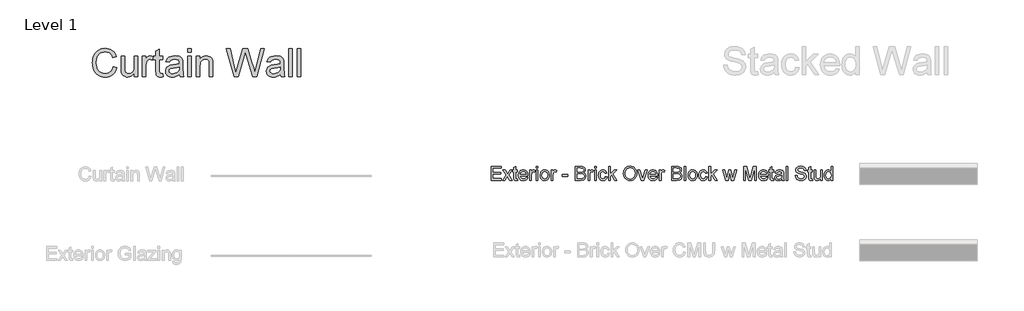
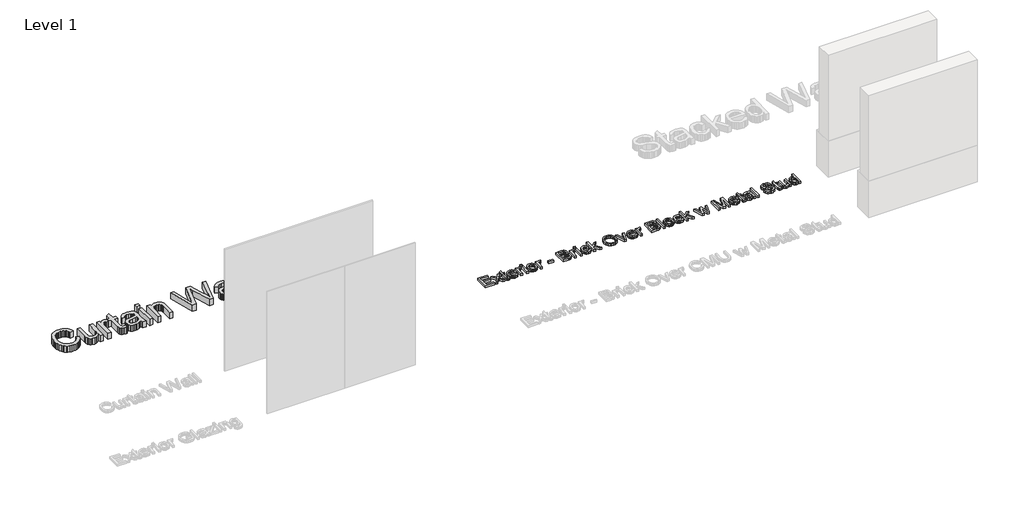
# One storey, part 41 of 42: 2 proxies.
"""IFC4 building model written with IfcOpenShell, lengths in millimetres."""

from ifc_helpers import new_model, si_unit, origin, origin_with_axes, place, context, project, spatial, polyline, outline, extrude, element, save

model = new_model("IFC4")

# Units and contexts
model_context = context("Model", 3, world=origin())
ifc_project = project(units=[si_unit("LENGTHUNIT", "METRE", prefix="MILLI")], contexts=[model_context])

# Site, building, storey
site = spatial("IfcSite", under=ifc_project)
building = spatial("IfcBuilding", under=site)
storey = spatial("IfcBuildingStorey", under=building, Name="Level 1", Elevation=0.0)

# Proxies
placement = place(None, origin())
element("IfcBuildingElementProxy", 1, Name="24\" Arial", ObjectType="24\" Arial", at=placement, inside=storey, context=model_context, shape_type="SweptSolid", body=[
    extrude(outline(polyline([(19167.4000192, 19179.27223), (19243.5417927, 19159.641929), (19228.475165, 19112.2903341), (19208.4080154, 19070.9151993), (19183.3403441, 19035.5165244), (19153.2721511, 19006.0943095), (19118.8819458, 18982.9645728), (19080.8482376, 18966.4433323), (19039.1710266, 18956.530588), (18993.8503128, 18953.2263398), (18947.4188883, 18955.7266007), (18905.5325477, 18963.2273833), (18868.1912909, 18975.7286877), (18835.3951181, 18993.2305138), (18806.6932386, 19015.4726115), (18781.634862, 19042.1947305), (18760.2199882, 19073.3968708), (18742.4486172, 19109.0790325), (18728.4927001, 19147.6983036), (18718.5241879, 19187.7117723), (18712.5430806, 19229.1194384), (18710.5493781, 19271.921302), (18712.8033308, 19317.8461681), (18719.5651887, 19360.7409783), (18730.8349519, 19400.6057325), (18746.6126205, 19437.4404308), (18766.5449976, 19470.6362736), (18790.2788866, 19499.5844613), (18817.8142875, 19524.2849939), (18849.1512002, 19544.7378714), (18883.2253874, 19560.7757901), (18918.9726117, 19572.2314464), (18956.3928729, 19579.1048401), (18995.4861712, 19581.3959714), (19039.0362542, 19578.430978), (19078.9707183, 19569.5359978), (19115.2895635, 19554.711031), (19147.9927898, 19533.9560773), (19176.5413076, 19507.8195213), (19200.396027, 19476.8497472), (19219.5569482, 19441.046755), (19234.0240711, 19400.4105449), (19157.8822975, 19382.2673879), (19145.8921989, 19412.2101031), (19131.4854913, 19437.7936275), (19114.6621746, 19459.017961), (19095.4222489, 19475.8831036), (19073.6541784, 19488.7329573), (19049.2464273, 19497.9114243), (19022.1989956, 19503.4185045), (18992.5118832, 19505.2541978), (18958.3540441, 19503.2186695), (18927.1147252, 19497.1120844), (18898.7939263, 19486.9344425), (18873.3916477, 19472.6857439), (18851.2285545, 19455.0073195), (18832.6253124, 19434.5405), (18817.5819212, 19411.2852855), (18806.098381, 19385.2416759), (18791.542959, 19329.510954), (18786.6911516, 19272.0700164), (18792.4352454, 19201.7281046), (18799.6153626, 19170.1262943), (18809.6675267, 19140.9039144), (18822.754394, 19114.6418806), (18839.0386209, 19091.9211085), (18858.5202075, 19072.741598), (18881.1991537, 19057.1033492), (18905.9740435, 19044.9691835), (18931.7434609, 19036.3019223), (18958.5074058, 19031.1015656), (18986.2658783, 19029.3681134), (19019.3687746, 19031.7289545), (19049.8226956, 19038.8114779), (19077.6276414, 19050.6156835), (19102.7836118, 19067.1415713), (19124.6957494, 19088.3147842), (19142.7691965, 19114.060965), (19157.0039531, 19144.3801135), (19167.4000192, 19179.27223)])), origin_with_axes(), (0.0, 0.0, 1.0), 152.4),
    extrude(outline(polyline([(19624.2506603, 18962.7440615), (19624.2506603, 19039.6294071), (19596.7013175, 19001.8280652), (19564.6161854, 18974.8271066), (19527.995264, 18958.6265315), (19486.8385534, 18953.2263398), (19449.7528996, 18957.0185571), (19415.2325692, 18968.3952088), (19386.2704395, 18985.4973649), (19365.8593879, 19006.4660955), (19352.1218951, 19031.9334368), (19343.1804417, 19062.5314249), (19338.7190096, 19133.3194799), (19338.7190096, 19410.0769809), (19414.8607832, 19410.0769809), (19414.8607832, 19169.1596507), (19416.0133198, 19120.9761846), (19419.4709296, 19091.5307331), (19430.5687418, 19065.635838), (19449.5855959, 19045.9497691), (19475.2574194, 19033.5135273), (19506.32014, 19029.3681134), (19539.1674334, 19033.6064738), (19569.8955466, 19046.3215551), (19595.2327628, 19066.3422314), (19611.907365, 19092.4973768), (19621.1648365, 19128.3189582), (19624.2506603, 19177.3389428), (19624.2506603, 19410.0769809), (19700.3924338, 19410.0769809), (19700.3924338, 18962.7440615), (19624.2506603, 18962.7440615)])), origin_with_axes(), (0.0, 0.0, 1.0), 152.4),
    extrude(outline(polyline([(19805.0873724, 18962.7440615), (19805.0873724, 19410.0769809), (19871.7114243, 19410.0769809), (19871.7114243, 19343.8990723), (19896.3236577, 19382.2673879), (19919.0026039, 19404.8719769), (19941.7559073, 19415.9140212), (19966.5912124, 19419.5947026), (20004.5133847, 19413.7204838), (20043.0304147, 19396.0978272), (20017.600252, 19327.837917), (19990.8316598, 19339.5491761), (19964.0630675, 19343.4529291), (19941.3283534, 19339.6978905), (19921.0102483, 19328.4327746), (19904.5958963, 19310.5126892), (19893.5724413, 19286.7927422), (19884.3149698, 19244.2604234), (19881.2291459, 19197.8615301), (19881.2291459, 18962.7440615), (19805.0873724, 18962.7440615)])), origin_with_axes(), (0.0, 0.0, 1.0), 152.4),
    extrude(outline(polyline([(20252.4202918, 19026.2451109), (20261.9380135, 18960.5133455), (20231.7861686, 18955.0480913), (20204.9803978, 18953.2263398), (20168.4338337, 18956.3865209), (20141.1819196, 18965.867064), (20121.9234046, 18980.4782539), (20109.3570377, 18999.0303755), (20102.441818, 19030.892436), (20100.1367448, 19085.4334427), (20100.1367448, 19333.9352074), (20043.0304147, 19333.9352074), (20043.0304147, 19410.0769809), (20100.1367448, 19410.0769809), (20100.1367448, 19518.7872084), (20176.2785183, 19563.5502432), (20176.2785183, 19410.0769809), (20252.4202918, 19410.0769809), (20252.4202918, 19333.9352074), (20176.2785183, 19333.9352074), (20176.2785183, 19087.6641587), (20180.2938072, 19048.4035567), (20193.3063173, 19034.4987602), (20204.2925937, 19030.6507751), (20219.2569803, 19029.3681134), (20252.4202918, 19026.2451109)])), origin_with_axes(), (0.0, 0.0, 1.0), 152.4),
    extrude(outline(polyline([(20614.0937161, 19019.8503917), (20577.7144556, 18988.657546), (20540.2570158, 18968.2464944), (20500.8662887, 18956.9813785), (20458.6871666, 18953.2263398), (20424.7849304, 18955.4849398), (20395.0559921, 18962.2607397), (20369.5003517, 18973.5537396), (20348.1180091, 18989.3639394), (20331.2342773, 19008.6875169), (20319.1744688, 19030.52065), (20311.9385837, 19054.8633386), (20309.526622, 19081.7155827), (20313.1701248, 19113.2802144), (20324.1006333, 19141.9449152), (20340.9611286, 19166.4827915), (20362.3945917, 19185.6669492), (20387.5830934, 19200.1666034), (20415.7087046, 19210.6509687), (20481.5891844, 19222.1019776), (20559.4411735, 19234.1478441), (20613.6475728, 19248.2757122), (20614.0937161, 19265.229154), (20608.8515334, 19299.2103947), (20602.2988051, 19311.7953509), (20593.1249855, 19321.4431977), (20577.2683124, 19331.0724552), (20557.9540295, 19337.9504963), (20508.9526343, 19343.4529291), (20463.5947418, 19339.790837), (20431.9185743, 19328.8045606), (20410.3178075, 19308.4864555), (20395.1861172, 19276.8288773), (20319.0443437, 19286.346599), (20332.2613361, 19327.9866314), (20351.9845836, 19360.7037997), (20380.0544268, 19385.7249977), (20418.3112066, 19404.2771193), (20465.1004751, 19415.7653068), (20518.7677848, 19419.5947026), (20570.2415569, 19416.21145), (20611.0450708, 19406.0616921), (20641.8103626, 19390.7998767), (20663.1694685, 19372.0804514), (20677.3345152, 19348.9367727), (20686.5176295, 19320.4021969), (20690.2354896, 19253.7781451), (20690.2354896, 19159.0470714), (20694.102064, 19026.7656113), (20699.8275685, 18994.0670323), (20709.2709329, 18962.7440615), (20633.1291594, 18962.7440615), (20620.9345785, 18989.215225), (20614.0937161, 19019.8503917)]), holes=[polyline([(20614.0937161, 19172.1339387), (20562.935962, 19159.456036), (20491.2556205, 19148.7857777), (20425.7469267, 19136.4424824), (20408.7005384, 19128.0029401), (20396.0784036, 19116.3660382), (20388.2708975, 19102.4240631), (20385.6683955, 19087.0693011), (20391.3381321, 19064.4275335), (20408.3473417, 19045.8754119), (20436.3242385, 19033.494938), (20474.8970363, 19029.3681134), (20515.7934967, 19033.9224919), (20551.9310963, 19047.5856275), (20581.2278333, 19067.7178396), (20601.6017063, 19091.6794475), (20610.6361062, 19116.3660382), (20613.6475728, 19150.5703505), (20614.0937161, 19172.1339387)])]), origin_with_axes(), (0.0, 0.0, 1.0), 152.4),
    extrude(outline(polyline([(20794.9304282, 19495.7364762), (20794.9304282, 19571.8782497), (20871.0722017, 19571.8782497), (20871.0722017, 19495.7364762), (20794.9304282, 19495.7364762)])), origin_with_axes(), (0.0, 0.0, 1.0), 152.4),
    extrude(outline(polyline([(20794.9304282, 18962.7440615), (20794.9304282, 19410.0769809), (20871.0722017, 19410.0769809), (20871.0722017, 18962.7440615), (20794.9304282, 18962.7440615)])), origin_with_axes(), (0.0, 0.0, 1.0), 152.4),
    extrude(outline(polyline([(20985.2848619, 18962.7440615), (20985.2848619, 19410.0769809), (21061.4266355, 19410.0769809), (21061.4266355, 19347.6169324), (21087.8792096, 19379.1072069), (21119.6483236, 19401.6002601), (21156.7339775, 19415.096092), (21199.1361712, 19419.5947026), (21236.6679682, 19415.9697891), (21271.0395842, 19405.0950485), (21299.7042851, 19388.3274997), (21320.1153367, 19367.0241617), (21333.9643653, 19341.2408024), (21342.9429973, 19311.0331896), (21346.9582862, 19237.4195609), (21346.9582862, 18962.7440615), (21270.8165126, 18962.7440615), (21270.8165126, 19227.1582672), (21268.6229752, 19266.530405), (21262.042363, 19294.5258911), (21249.9035499, 19314.5837459), (21231.0354103, 19330.1429902), (21206.8507307, 19340.1254444), (21178.7622982, 19343.4529291), (21155.6418561, 19341.5847045), (21134.166567, 19335.9800304), (21114.3364311, 19326.6389071), (21096.1514482, 19313.5613344), (21080.9593426, 19295.2601684), (21070.1078386, 19270.248265), (21063.5969363, 19238.5256243), (21061.4266355, 19200.0922462), (21061.4266355, 18962.7440615), (20985.2848619, 18962.7440615)])), origin_with_axes(), (0.0, 0.0, 1.0), 152.4),
    extrude(outline(polyline([(21808.1216449, 18962.7440615), (21642.0076585, 19571.8782497), (21720.5288625, 19571.8782497), (21816.8957946, 19171.5390811), (21846.6386749, 19047.9574135), (21878.4635568, 19157.2624986), (21999.2196507, 19571.8782497), (22112.3913102, 19571.8782497), (22200.132807, 19271.3264444), (22237.7203719, 19159.7906434), (22265.4184292, 19047.9574135), (22294.2690231, 19167.9699355), (22391.5282416, 19571.8782497), (22470.0494455, 19571.8782497), (22303.7867448, 18962.7440615), (22222.4399672, 18962.7440615), (22076.402425, 19432.68157), (22056.028552, 19498.264621), (22033.1265342, 19419.2972738), (21900.027145, 18962.7440615), (21808.1216449, 18962.7440615)])), origin_with_axes(), (0.0, 0.0, 1.0), 152.4),
    extrude(outline(polyline([(22822.205148, 19019.8503917), (22785.8258876, 18988.657546), (22748.3684478, 18968.2464944), (22708.9777207, 18956.9813785), (22666.7985986, 18953.2263398), (22632.8963624, 18955.4849398), (22603.1674241, 18962.2607397), (22577.6117837, 18973.5537396), (22556.2294411, 18989.3639394), (22539.3457093, 19008.6875169), (22527.2859008, 19030.52065), (22520.0500157, 19054.8633386), (22517.638054, 19081.7155827), (22521.2815568, 19113.2802144), (22532.2120653, 19141.9449152), (22549.0725606, 19166.4827915), (22570.5060237, 19185.6669492), (22595.6945254, 19200.1666034), (22623.8201366, 19210.6509687), (22689.7006164, 19222.1019776), (22767.5526055, 19234.1478441), (22821.7590048, 19248.2757122), (22822.205148, 19265.229154), (22816.9629654, 19299.2103947), (22810.4102371, 19311.7953509), (22801.2364174, 19321.4431977), (22785.3797444, 19331.0724552), (22766.0654615, 19337.9504963), (22717.0640663, 19343.4529291), (22671.7061738, 19339.790837), (22640.0300063, 19328.8045606), (22618.4292395, 19308.4864555), (22603.2975492, 19276.8288773), (22527.1557757, 19286.346599), (22540.3727681, 19327.9866314), (22560.0960156, 19360.7037997), (22588.1658588, 19385.7249977), (22626.4226386, 19404.2771193), (22673.2119071, 19415.7653068), (22726.8792167, 19419.5947026), (22778.3529889, 19416.21145), (22819.1565028, 19406.0616921), (22849.9217946, 19390.7998767), (22871.2809005, 19372.0804514), (22885.4459472, 19348.9367727), (22894.6290615, 19320.4021969), (22898.3469216, 19253.7781451), (22898.3469216, 19159.0470714), (22902.213496, 19026.7656113), (22907.9390005, 18994.0670323), (22917.3823649, 18962.7440615), (22841.2405914, 18962.7440615), (22829.0460105, 18989.215225), (22822.205148, 19019.8503917)]), holes=[polyline([(22822.205148, 19172.1339387), (22771.047394, 19159.456036), (22699.3670525, 19148.7857777), (22633.8583587, 19136.4424824), (22616.8119704, 19128.0029401), (22604.1898356, 19116.3660382), (22596.3823295, 19102.4240631), (22593.7798275, 19087.0693011), (22599.449564, 19064.4275335), (22616.4587737, 19045.8754119), (22644.4356705, 19033.494938), (22683.0084683, 19029.3681134), (22723.9049287, 19033.9224919), (22760.0425283, 19047.5856275), (22789.3392653, 19067.7178396), (22809.7131383, 19091.6794475), (22818.7475382, 19116.3660382), (22821.7590048, 19150.5703505), (22822.205148, 19172.1339387)])]), origin_with_axes(), (0.0, 0.0, 1.0), 152.4),
    extrude(outline(polyline([(23003.0418601, 18962.7440615), (23003.0418601, 19571.8782497), (23079.1836337, 19571.8782497), (23079.1836337, 18962.7440615), (23003.0418601, 18962.7440615)])), origin_with_axes(), (0.0, 0.0, 1.0), 152.4),
    extrude(outline(polyline([(23193.3962939, 18962.7440615), (23193.3962939, 19571.8782497), (23269.5380675, 19571.8782497), (23269.5380675, 18962.7440615), (23193.3962939, 18962.7440615)])), origin_with_axes(), (0.0, 0.0, 1.0), 152.4),
])
element("IfcBuildingElementProxy", 2, Name="8\" Arial", ObjectType="8\" Arial", at=placement, inside=storey, context=model_context, shape_type="SweptSolid", body=[
    extrude(outline(polyline([(27431.9881133, 16690.4462247), (27431.9881133, 16995.0133187), (27650.8957121, 16995.0133187), (27650.8957121, 16956.942432), (27470.059, 16956.942432), (27470.059, 16866.5240759), (27641.3779905, 16866.5240759), (27641.3779905, 16828.4531892), (27470.059, 16828.4531892), (27470.059, 16728.5171114), (27655.654573, 16728.5171114), (27655.654573, 16690.4462247), (27431.9881133, 16690.4462247)])), origin_with_axes(), (0.0, 0.0, 1.0), 50.8),
    extrude(outline(polyline([(27684.2077381, 16690.4462247), (27765.5545156, 16802.8743121), (27688.9665989, 16914.1126844), (27734.7706345, 16914.1126844), (27771.7261633, 16860.5754999), (27788.9770338, 16835.2940516), (27803.9228312, 16855.9653534), (27846.0090068, 16914.1126844), (27891.8130424, 16914.1126844), (27811.3585513, 16802.8743121), (27888.8387544, 16690.4462247), (27843.0347188, 16690.4462247), (27796.4127539, 16758.0369201), (27787.8616758, 16770.3802154), (27730.0117737, 16690.4462247), (27684.2077381, 16690.4462247)])), origin_with_axes(), (0.0, 0.0, 1.0), 50.8),
    extrude(outline(polyline([(28003.0514147, 16722.1967494), (28007.8102755, 16689.3308667), (27979.3314676, 16685.6873638), (27961.0581856, 16687.2674543), (27947.4322285, 16692.0077259), (27937.802971, 16699.3133208), (27931.5197876, 16708.5893816), (27928.0621778, 16724.5204119), (27926.9096411, 16751.7909152), (27926.9096411, 16876.0417976), (27898.3564761, 16876.0417976), (27898.3564761, 16914.1126844), (27926.9096411, 16914.1126844), (27926.9096411, 16968.4677981), (27964.9805279, 16990.8493155), (27964.9805279, 16914.1126844), (28003.0514147, 16914.1126844), (28003.0514147, 16876.0417976), (27964.9805279, 16876.0417976), (27964.9805279, 16752.9062732), (27966.9881723, 16733.2759723), (27973.4944274, 16726.323574), (27986.4697589, 16723.7582506), (28003.0514147, 16722.1967494)])), origin_with_axes(), (0.0, 0.0, 1.0), 50.8),
    extrude(outline(polyline([(28197.7185661, 16757.0702765), (28235.0458808, 16752.3114156), (28221.5965222, 16724.1858045), (28200.1351751, 16703.161306), (28171.1451615, 16690.0558494), (28135.1098031, 16685.6873638), (28111.4874499, 16687.5718541), (28090.4397148, 16693.225325), (28071.9665977, 16702.6477766), (28056.0680988, 16715.8392087), (28043.2833076, 16732.4324828), (28034.1513139, 16752.0604601), (28028.6721176, 16774.7231407), (28026.8457189, 16800.4205245), (28028.6907069, 16826.9892818), (28034.2256711, 16850.4071527), (28043.4506113, 16870.6741372), (28056.3655276, 16887.7902353), (28072.2222006, 16901.3883084), (28090.2724111, 16911.1012177), (28110.516159, 16916.9289633), (28132.9534443, 16918.8715452), (28154.6680706, 16916.9336107), (28174.3053425, 16911.119807), (28191.8652602, 16901.4301343), (28207.3478236, 16887.8645925), (28219.986224, 16870.785673), (28229.0136529, 16850.5558671), (28234.4301103, 16827.1751748), (28236.2355961, 16800.6435961), (28236.0125245, 16790.3823024), (28064.9166056, 16790.3823024), (28071.5065126, 16761.8849052), (28086.8148013, 16740.9347639), (28108.9081845, 16728.0523789), (28135.8533751, 16723.7582506), (28156.1157123, 16725.7473057), (28173.1806899, 16731.7144711), (28187.0483078, 16742.0315326), (28197.7185661, 16757.0702765)]), holes=[polyline([(28064.9166056, 16828.4531892), (28198.1647093, 16828.4531892), (28193.0154732, 16848.566812), (28182.9214832, 16862.9549303), (28160.7258587, 16876.3392264), (28132.8047299, 16880.8006585), (28107.142201, 16877.2408075), (28085.9225148, 16866.5612545), (28071.1719052, 16849.9145362), (28064.9166056, 16828.4531892)])]), origin_with_axes(), (0.0, 0.0, 1.0), 50.8),
    extrude(outline(polyline([(28274.3064828, 16690.4462247), (28274.3064828, 16914.1126844), (28307.6185087, 16914.1126844), (28307.6185087, 16881.0237301), (28319.9246254, 16900.2078878), (28331.2640986, 16911.5101823), (28342.6407503, 16917.0312045), (28355.0584028, 16918.8715452), (28374.019489, 16915.9344358), (28393.2780039, 16907.1231075), (28380.5629226, 16872.9931524), (28367.1786265, 16878.8487819), (28353.7943304, 16880.8006585), (28342.4269733, 16878.9231391), (28332.2679208, 16873.2905812), (28324.0607447, 16864.3305385), (28318.5490172, 16852.470565), (28313.9202815, 16831.2044056), (28312.3773696, 16808.004959), (28312.3773696, 16690.4462247), (28274.3064828, 16690.4462247)])), origin_with_axes(), (0.0, 0.0, 1.0), 50.8),
    extrude(outline(polyline([(28417.0723082, 16956.942432), (28417.0723082, 16995.0133187), (28455.1431949, 16995.0133187), (28455.1431949, 16956.942432), (28417.0723082, 16956.942432)])), origin_with_axes(), (0.0, 0.0, 1.0), 50.8),
    extrude(outline(polyline([(28417.0723082, 16690.4462247), (28417.0723082, 16914.1126844), (28455.1431949, 16914.1126844), (28455.1431949, 16690.4462247), (28417.0723082, 16690.4462247)])), origin_with_axes(), (0.0, 0.0, 1.0), 50.8),
    extrude(outline(polyline([(28502.7318034, 16802.2794545), (28504.7905684, 16831.2462315), (28510.9668633, 16856.2070143), (28521.2606883, 16877.1618029), (28535.6720433, 16894.1105974), (28550.1809921, 16904.9435121), (28566.1956742, 16912.6813083), (28583.7160896, 16917.323986), (28602.7422383, 16918.8715452), (28623.7458238, 16916.9870549), (28642.7371176, 16911.333584), (28659.7161197, 16901.9111325), (28674.68283, 16888.7197003), (28686.8983239, 16872.2054308), (28695.6236766, 16852.814467), (28700.8588883, 16830.5468091), (28702.6039589, 16805.4024569), (28699.518135, 16766.9411949), (28690.2606635, 16737.6630471), (28675.1010892, 16715.7369675), (28654.308957, 16699.3319101), (28629.6130717, 16689.0985004), (28602.7422383, 16685.6873638), (28581.4319293, 16687.5648831), (28562.2640372, 16693.1974411), (28545.2385619, 16702.5850377), (28530.3555034, 16715.7276729), (28518.2701347, 16732.4022752), (28509.6377284, 16752.3857728), (28504.4582846, 16775.678166), (28502.7318034, 16802.2794545)]), holes=[polyline([(28540.8026901, 16802.3538117), (28545.2083543, 16767.8985438), (28558.4253467, 16743.351373), (28578.3158979, 16728.6565312), (28602.7422383, 16723.7582506), (28627.0570429, 16728.6844151), (28646.9104155, 16743.4629088), (28660.127408, 16768.3353924), (28664.5330721, 16803.5435269), (28660.099524, 16836.9949726), (28646.7988797, 16861.2075361), (28626.9176232, 16875.9023779), (28602.7422383, 16880.8006585), (28578.3158979, 16875.9209672), (28558.4253467, 16861.2818933), (28545.2083543, 16836.7904903), (28540.8026901, 16802.3538117)])]), origin_with_axes(), (0.0, 0.0, 1.0), 50.8),
    extrude(outline(polyline([(28745.4337065, 16690.4462247), (28745.4337065, 16914.1126844), (28778.7457324, 16914.1126844), (28778.7457324, 16881.0237301), (28791.0518491, 16900.2078878), (28802.3913222, 16911.5101823), (28813.7679739, 16917.0312045), (28826.1856264, 16918.8715452), (28845.1467126, 16915.9344358), (28864.4052276, 16907.1231075), (28851.6901463, 16872.9931524), (28838.3058501, 16878.8487819), (28824.921554, 16880.8006585), (28813.5541969, 16878.9231391), (28803.3951444, 16873.2905812), (28795.1879684, 16864.3305385), (28789.6762409, 16852.470565), (28785.0475051, 16831.2044056), (28783.5045932, 16808.004959), (28783.5045932, 16690.4462247), (28745.4337065, 16690.4462247)])), origin_with_axes(), (0.0, 0.0, 1.0), 50.8),
    extrude(outline(polyline([(28988.1356095, 16780.8645807), (28988.1356095, 16818.9354675), (29107.1071307, 16818.9354675), (29107.1071307, 16780.8645807), (28988.1356095, 16780.8645807)])), origin_with_axes(), (0.0, 0.0, 1.0), 50.8),
    extrude(outline(polyline([(29273.6672602, 16690.4462247), (29273.6672602, 16995.0133187), (29389.8875649, 16995.0133187), (29421.8518666, 16992.7733081), (29446.8080021, 16986.053276), (29465.9363919, 16974.685919), (29480.4174568, 16958.5039332), (29489.5355085, 16939.4684898), (29492.5748591, 16919.54076), (29490.0188303, 16901.2024154), (29482.350744, 16883.9608395), (29469.5148322, 16868.8756224), (29451.4553271, 16857.0063542), (29473.02821, 16845.7412383), (29488.9685349, 16828.6019036), (29498.8115693, 16806.7222973), (29502.0925808, 16781.2363667), (29499.8525701, 16759.9980913), (29493.1325381, 16740.3027277), (29483.1036107, 16723.5537683), (29470.9369137, 16711.1547051), (29456.0375896, 16702.1760731), (29437.8107808, 16695.6884073), (29388.9952785, 16690.4462247), (29273.6672602, 16690.4462247)]), holes=[polyline([(29311.738147, 16871.2829368), (29381.2621296, 16871.2829368), (29421.8611612, 16874.5546536), (29436.0726812, 16880.1965062), (29446.2875017, 16888.6453431), (29452.4498547, 16899.7710393), (29454.5039723, 16913.4434696), (29452.5892744, 16926.7162299), (29446.8451807, 16938.2787746), (29437.5319413, 16947.3038798), (29424.9098065, 16952.9643217), (29375.9827684, 16956.942432), (29311.738147, 16956.942432), (29311.738147, 16871.2829368)]), polyline([(29311.738147, 16728.5171114), (29389.8132077, 16728.5171114), (29418.068944, 16730.0042554), (29441.974784, 16738.2950833), (29457.8128678, 16755.2113465), (29462.4694875, 16767.1642665), (29464.021694, 16780.8645807), (29462.1999426, 16796.7770217), (29456.7346884, 16810.4587466), (29447.1890827, 16821.1568888), (29433.1262771, 16828.1185818), (29413.207842, 16831.9386829), (29386.0953477, 16833.21205), (29311.738147, 16833.21205), (29311.738147, 16728.5171114)])]), origin_with_axes(), (0.0, 0.0, 1.0), 50.8),
    extrude(outline(polyline([(29549.6811892, 16690.4462247), (29549.6811892, 16914.1126844), (29582.9932151, 16914.1126844), (29582.9932151, 16881.0237301), (29595.2993319, 16900.2078878), (29606.638805, 16911.5101823), (29618.0154567, 16917.0312045), (29630.4331092, 16918.8715452), (29649.3941954, 16915.9344358), (29668.6527104, 16907.1231075), (29655.937629, 16872.9931524), (29642.5533329, 16878.8487819), (29629.1690368, 16880.8006585), (29617.8016797, 16878.9231391), (29607.6426272, 16873.2905812), (29599.4354511, 16864.3305385), (29593.9237236, 16852.470565), (29589.2949879, 16831.2044056), (29587.752076, 16808.004959), (29587.752076, 16690.4462247), (29549.6811892, 16690.4462247)])), origin_with_axes(), (0.0, 0.0, 1.0), 50.8),
    extrude(outline(polyline([(29692.4470146, 16690.4462247), (29692.4470146, 16914.1126844), (29730.5179013, 16914.1126844), (29730.5179013, 16690.4462247), (29692.4470146, 16690.4462247)])), origin_with_axes(), (0.0, 0.0, 1.0), 50.8),
    extrude(outline(polyline([(29692.4470146, 16956.942432), (29692.4470146, 16995.0133187), (29730.5179013, 16995.0133187), (29730.5179013, 16956.942432), (29692.4470146, 16956.942432)])), origin_with_axes(), (0.0, 0.0, 1.0), 50.8),
    extrude(outline(polyline([(29930.3900568, 16771.346859), (29968.4609436, 16766.5879982), (29957.8464532, 16732.7275879), (29937.9001341, 16707.1394162), (29910.4995056, 16691.0503769), (29877.5220871, 16685.6873638), (29856.1699522, 16687.5579121), (29837.0252967, 16693.1695571), (29820.0881206, 16702.5222988), (29805.3584238, 16715.6161371), (29793.4357114, 16732.2047638), (29784.9194883, 16752.0418708), (29779.8097544, 16775.1274579), (29778.1065098, 16801.4615253), (29781.0157353, 16835.3405249), (29789.7434117, 16864.7023245), (29804.4289588, 16888.4129769), (29825.2117964, 16905.3385347), (29850.0749854, 16915.4882926), (29877.0015867, 16918.8715452), (29909.1703707, 16914.2242202), (29934.8886675, 16900.282245), (29953.3385479, 16877.7891918), (29963.7020827, 16847.4886325), (29925.631196, 16842.7297717), (29918.725271, 16859.3393114), (29907.9713608, 16871.2457582), (29893.9643231, 16878.4119334), (29877.2990155, 16880.8006585), (29852.6960767, 16876.0975655), (29833.1680169, 16861.9882867), (29820.4250516, 16837.7106606), (29816.1773965, 16802.5025261), (29820.3321051, 16766.8203644), (29832.7962309, 16742.4590866), (29851.971094, 16728.4334596), (29876.2580147, 16723.7582506), (29895.9719675, 16726.6767707), (29912.135364, 16735.4323311), (29923.8930964, 16750.2480033), (29930.3900568, 16771.346859)])), origin_with_axes(), (0.0, 0.0, 1.0), 50.8),
    extrude(outline(polyline([(30001.7729695, 16690.4462247), (30001.7729695, 16995.0133187), (30039.8438562, 16995.0133187), (30039.8438562, 16831.35312), (30125.2059227, 16914.1126844), (30177.8508207, 16914.1126844), (30091.4477535, 16830.3121192), (30182.6096816, 16690.4462247), (30138.1440756, 16690.4462247), (30064.1586609, 16803.8409557), (30039.8438562, 16780.2697231), (30039.8438562, 16690.4462247), (30001.7729695, 16690.4462247)])), origin_with_axes(), (0.0, 0.0, 1.0), 50.8),
    extrude(outline(polyline([(30325.3755069, 16838.7144829), (30327.9129464, 16874.4384705), (30335.5252648, 16906.0635174), (30348.2124622, 16933.5896236), (30365.9745385, 16957.0167892), (30387.7472563, 16975.7222725), (30412.4663783, 16989.083332), (30440.1319042, 16997.0999677), (30470.7438343, 16999.7721796), (30510.6922404, 16994.7530685), (30546.5138218, 16979.6957354), (30576.2567021, 16955.6597703), (30597.9690047, 16923.7047633), (30611.241765, 16885.3736263), (30615.6660185, 16842.2092713), (30611.0093988, 16798.468648), (30597.0395397, 16759.5984213), (30574.5278972, 16727.5876464), (30544.2459272, 16704.4253784), (30508.7310692, 16690.3718675), (30470.5207627, 16685.6873638), (30429.9589097, 16690.8644839), (30393.932846, 16706.3958442), (30364.2643229, 16730.8779525), (30342.7750919, 16762.9073167), (30329.7254032, 16799.7606043), (30325.3755069, 16838.7144829)]), holes=[polyline([(30363.4463937, 16838.3426969), (30365.3494733, 16813.1030745), (30371.0587121, 16790.6983205), (30380.5741101, 16771.1284347), (30393.8956674, 16754.3934173), (30410.0892715, 16740.9905318), (30428.2208102, 16731.4170422), (30448.2902834, 16725.6729485), (30470.2976911, 16723.7582506), (30492.6815322, 16725.6915378), (30512.988019, 16731.4913994), (30531.2171514, 16741.1578355), (30547.3689296, 16754.6908461), (30560.592893, 16771.7790603), (30570.0385812, 16792.1111073), (30575.7059941, 16815.6869873), (30577.5951317, 16842.5067001), (30574.3605935, 16876.2091013), (30564.6569788, 16905.3385347), (30548.7352432, 16929.1607229), (30526.8463422, 16946.9413885), (30500.4402413, 16958.0113167), (30470.9669059, 16961.7012928), (30449.7239831, 16959.923691), (30430.0146776, 16954.5908855), (30411.8389894, 16945.7028764), (30395.1969184, 16933.2596635), (30381.3060638, 16916.6617422), (30371.3840249, 16895.3096072), (30365.4308015, 16869.2032588), (30363.4463937, 16838.3426969)])]), origin_with_axes(), (0.0, 0.0, 1.0), 50.8),
    extrude(outline(polyline([(30718.130241, 16690.4462247), (30639.4603227, 16914.1126844), (30679.7619255, 16914.1126844), (30727.4248911, 16780.1210087), (30741.7758309, 16735.0605451), (30755.8293418, 16777.5928639), (30803.7897362, 16914.1126844), (30844.091339, 16914.1126844), (30766.3880643, 16690.4462247), (30718.130241, 16690.4462247)])), origin_with_axes(), (0.0, 0.0, 1.0), 50.8),
    extrude(outline(polyline([(31033.9996296, 16757.0702765), (31071.3269444, 16752.3114156), (31057.8775857, 16724.1858045), (31036.4162386, 16703.161306), (31007.426225, 16690.0558494), (30971.3908666, 16685.6873638), (30947.7685134, 16687.5718541), (30926.7207783, 16693.225325), (30908.2476612, 16702.6477766), (30892.3491623, 16715.8392087), (30879.5643711, 16732.4324828), (30870.4323774, 16752.0604601), (30864.9531811, 16774.7231407), (30863.1267824, 16800.4205245), (30864.9717704, 16826.9892818), (30870.5067346, 16850.4071527), (30879.7316748, 16870.6741372), (30892.6465911, 16887.7902353), (30908.5032641, 16901.3883084), (30926.5534746, 16911.1012177), (30946.7972225, 16916.9289633), (30969.2345078, 16918.8715452), (30990.9491341, 16916.9336107), (31010.586406, 16911.119807), (31028.1463237, 16901.4301343), (31043.6288871, 16887.8645925), (31056.2672876, 16870.785673), (31065.2947165, 16850.5558671), (31070.7111738, 16827.1751748), (31072.5166596, 16800.6435961), (31072.293588, 16790.3823024), (30901.1976692, 16790.3823024), (30907.7875761, 16761.8849052), (30923.0958648, 16740.9347639), (30945.189248, 16728.0523789), (30972.1344386, 16723.7582506), (30992.3967758, 16725.7473057), (31009.4617534, 16731.7144711), (31023.3293713, 16742.0315326), (31033.9996296, 16757.0702765)]), holes=[polyline([(30901.1976692, 16828.4531892), (31034.4457728, 16828.4531892), (31029.2965367, 16848.566812), (31019.2025467, 16862.9549303), (30997.0069223, 16876.3392264), (30969.0857934, 16880.8006585), (30943.4232645, 16877.2408075), (30922.2035784, 16866.5612545), (30907.4529687, 16849.9145362), (30901.1976692, 16828.4531892)])]), origin_with_axes(), (0.0, 0.0, 1.0), 50.8),
    extrude(outline(polyline([(31110.5875463, 16690.4462247), (31110.5875463, 16914.1126844), (31143.8995722, 16914.1126844), (31143.8995722, 16881.0237301), (31156.205689, 16900.2078878), (31167.5451621, 16911.5101823), (31178.9218138, 16917.0312045), (31191.3394663, 16918.8715452), (31210.3005525, 16915.9344358), (31229.5590675, 16907.1231075), (31216.8439861, 16872.9931524), (31203.45969, 16878.8487819), (31190.0753939, 16880.8006585), (31178.7080368, 16878.9231391), (31168.5489843, 16873.2905812), (31160.3418082, 16864.3305385), (31154.8300807, 16852.470565), (31150.201345, 16831.2044056), (31148.6584331, 16808.004959), (31148.6584331, 16690.4462247), (31110.5875463, 16690.4462247)])), origin_with_axes(), (0.0, 0.0, 1.0), 50.8),
    extrude(outline(polyline([(31377.0837536, 16690.4462247), (31377.0837536, 16995.0133187), (31493.3040583, 16995.0133187), (31525.26836, 16992.7733081), (31550.2244955, 16986.053276), (31569.3528854, 16974.685919), (31583.8339502, 16958.5039332), (31592.9520019, 16939.4684898), (31595.9913525, 16919.54076), (31593.4353237, 16901.2024154), (31585.7672374, 16883.9608395), (31572.9313256, 16868.8756224), (31554.8718205, 16857.0063542), (31576.4447034, 16845.7412383), (31592.3850283, 16828.6019036), (31602.2280627, 16806.7222973), (31605.5090742, 16781.2363667), (31603.2690635, 16759.9980913), (31596.5490315, 16740.3027277), (31586.5201041, 16723.5537683), (31574.3534071, 16711.1547051), (31559.454083, 16702.1760731), (31541.2272742, 16695.6884073), (31492.4117719, 16690.4462247), (31377.0837536, 16690.4462247)]), holes=[polyline([(31415.1546404, 16728.5171114), (31493.2297011, 16728.5171114), (31521.4854374, 16730.0042554), (31545.3912774, 16738.2950833), (31561.2293612, 16755.2113465), (31565.8859809, 16767.1642665), (31567.4381874, 16780.8645807), (31565.616436, 16796.7770217), (31560.1511818, 16810.4587466), (31550.6055761, 16821.1568888), (31536.5427705, 16828.1185818), (31516.6243354, 16831.9386829), (31489.5118411, 16833.21205), (31415.1546404, 16833.21205), (31415.1546404, 16728.5171114)]), polyline([(31415.1546404, 16871.2829368), (31484.6786231, 16871.2829368), (31525.2776546, 16874.5546536), (31539.4891746, 16880.1965062), (31549.7039951, 16888.6453431), (31555.8663481, 16899.7710393), (31557.9204657, 16913.4434696), (31556.0057678, 16926.7162299), (31550.2616741, 16938.2787746), (31540.9484347, 16947.3038798), (31528.3262999, 16952.9643217), (31479.3992618, 16956.942432), (31415.1546404, 16956.942432), (31415.1546404, 16871.2829368)])]), origin_with_axes(), (0.0, 0.0, 1.0), 50.8),
    extrude(outline(polyline([(31653.0976826, 16690.4462247), (31653.0976826, 16995.0133187), (31691.1685694, 16995.0133187), (31691.1685694, 16690.4462247), (31653.0976826, 16690.4462247)])), origin_with_axes(), (0.0, 0.0, 1.0), 50.8),
    extrude(outline(polyline([(31738.7571778, 16802.2794545), (31740.8159428, 16831.2462315), (31746.9922378, 16856.2070143), (31757.2860628, 16877.1618029), (31771.6974178, 16894.1105974), (31786.2063665, 16904.9435121), (31802.2210486, 16912.6813083), (31819.7414641, 16917.323986), (31838.7676128, 16918.8715452), (31859.7711983, 16916.9870549), (31878.7624921, 16911.333584), (31895.7414942, 16901.9111325), (31910.7082045, 16888.7197003), (31922.9236983, 16872.2054308), (31931.6490511, 16852.814467), (31936.8842628, 16830.5468091), (31938.6293333, 16805.4024569), (31935.5435095, 16766.9411949), (31926.286038, 16737.6630471), (31911.1264637, 16715.7369675), (31890.3343315, 16699.3319101), (31865.6384462, 16689.0985004), (31838.7676128, 16685.6873638), (31817.4573038, 16687.5648831), (31798.2894117, 16693.1974411), (31781.2639364, 16702.5850377), (31766.3808779, 16715.7276729), (31754.2955091, 16732.4022752), (31745.6631029, 16752.3857728), (31740.4836591, 16775.678166), (31738.7571778, 16802.2794545)]), holes=[polyline([(31776.8280646, 16802.3538117), (31781.2337287, 16767.8985438), (31794.4507212, 16743.351373), (31814.3412724, 16728.6565312), (31838.7676128, 16723.7582506), (31863.0824174, 16728.6844151), (31882.93579, 16743.4629088), (31896.1527824, 16768.3353924), (31900.5584466, 16803.5435269), (31896.1248985, 16836.9949726), (31882.8242542, 16861.2075361), (31862.9429977, 16875.9023779), (31838.7676128, 16880.8006585), (31814.3412724, 16875.9209672), (31794.4507212, 16861.2818933), (31781.2337287, 16836.7904903), (31776.8280646, 16802.3538117)])]), origin_with_axes(), (0.0, 0.0, 1.0), 50.8),
    extrude(outline(polyline([(32124.2249063, 16771.346859), (32162.295793, 16766.5879982), (32151.6813026, 16732.7275879), (32131.7349835, 16707.1394162), (32104.3343551, 16691.0503769), (32071.3569366, 16685.6873638), (32050.0048017, 16687.5579121), (32030.8601461, 16693.1695571), (32013.92297, 16702.5222988), (31999.1932733, 16715.6161371), (31987.2705609, 16732.2047638), (31978.7543378, 16752.0418708), (31973.6446039, 16775.1274579), (31971.9413592, 16801.4615253), (31974.8505847, 16835.3405249), (31983.5782612, 16864.7023245), (31998.2638083, 16888.4129769), (32019.0466459, 16905.3385347), (32043.9098349, 16915.4882926), (32070.8364362, 16918.8715452), (32103.0052201, 16914.2242202), (32128.7235169, 16900.282245), (32147.1733973, 16877.7891918), (32157.5369322, 16847.4886325), (32119.4660454, 16842.7297717), (32112.5601204, 16859.3393114), (32101.8062103, 16871.2457582), (32087.7991726, 16878.4119334), (32071.133865, 16880.8006585), (32046.5309262, 16876.0975655), (32027.0028664, 16861.9882867), (32014.2599011, 16837.7106606), (32010.012246, 16802.5025261), (32014.1669546, 16766.8203644), (32026.6310804, 16742.4590866), (32045.8059435, 16728.4334596), (32070.0928642, 16723.7582506), (32089.806817, 16726.6767707), (32105.9702135, 16735.4323311), (32117.7279459, 16750.2480033), (32124.2249063, 16771.346859)])), origin_with_axes(), (0.0, 0.0, 1.0), 50.8),
    extrude(outline(polyline([(32195.6078189, 16690.4462247), (32195.6078189, 16995.0133187), (32233.6787057, 16995.0133187), (32233.6787057, 16831.35312), (32319.0407721, 16914.1126844), (32371.6856702, 16914.1126844), (32285.282603, 16830.3121192), (32376.4445311, 16690.4462247), (32331.978925, 16690.4462247), (32257.9935103, 16803.8409557), (32233.6787057, 16780.2697231), (32233.6787057, 16690.4462247), (32195.6078189, 16690.4462247)])), origin_with_axes(), (0.0, 0.0, 1.0), 50.8),
    extrude(outline(polyline([(32565.8323212, 16690.4462247), (32497.7954826, 16914.1126844), (32537.3535134, 16914.1126844), (32575.9449005, 16783.6157971), (32587.4702666, 16736.9938323), (32596.9136311, 16781.9055815), (32627.623155, 16914.1126844), (32672.9810474, 16914.1126844), (32703.5418569, 16782.2773675), (32711.9442206, 16741.6039787), (32723.9900871, 16784.5080835), (32762.6558315, 16914.1126844), (32802.3625767, 16914.1126844), (32733.8052376, 16690.4462247), (32687.7781304, 16690.4462247), (32658.5557505, 16821.6123267), (32650.0790296, 16862.5087871), (32612.3799289, 16690.4462247), (32565.8323212, 16690.4462247)])), origin_with_axes(), (0.0, 0.0, 1.0), 50.8),
    extrude(outline(polyline([(32952.2666933, 16690.4462247), (32952.2666933, 16995.0133187), (33017.7753871, 16995.0133187), (33080.0867213, 16780.3440803), (33092.6530882, 16735.5066883), (33106.2604559, 16784.0619403), (33167.5307893, 16995.0133187), (33233.0394831, 16995.0133187), (33233.0394831, 16690.4462247), (33194.9685964, 16690.4462247), (33194.9685964, 16956.942432), (33118.4550368, 16690.4462247), (33066.8511396, 16690.4462247), (32990.33758, 16956.942432), (32990.33758, 16690.4462247), (32952.2666933, 16690.4462247)])), origin_with_axes(), (0.0, 0.0, 1.0), 50.8),
    extrude(outline(polyline([(33451.5009388, 16757.0702765), (33488.8282535, 16752.3114156), (33475.3788949, 16724.1858045), (33453.9175478, 16703.161306), (33424.9275342, 16690.0558494), (33388.8921758, 16685.6873638), (33365.2698226, 16687.5718541), (33344.2220875, 16693.225325), (33325.7489704, 16702.6477766), (33309.8504714, 16715.8392087), (33297.0656802, 16732.4324828), (33287.9336865, 16752.0604601), (33282.4544903, 16774.7231407), (33280.6280916, 16800.4205245), (33282.4730796, 16826.9892818), (33288.0080437, 16850.4071527), (33297.2329839, 16870.6741372), (33310.1479002, 16887.7902353), (33326.0045733, 16901.3883084), (33344.0547838, 16911.1012177), (33364.2985317, 16916.9289633), (33386.735817, 16918.8715452), (33408.4504432, 16916.9336107), (33428.0877152, 16911.119807), (33445.6476329, 16901.4301343), (33461.1301963, 16887.8645925), (33473.7685967, 16870.785673), (33482.7960256, 16850.5558671), (33488.212483, 16827.1751748), (33490.0179687, 16800.6435961), (33489.7948971, 16790.3823024), (33318.6989783, 16790.3823024), (33325.2888852, 16761.8849052), (33340.5971739, 16740.9347639), (33362.6905572, 16728.0523789), (33389.6357478, 16723.7582506), (33409.898085, 16725.7473057), (33426.9630625, 16731.7144711), (33440.8306805, 16742.0315326), (33451.5009388, 16757.0702765)]), holes=[polyline([(33318.6989783, 16828.4531892), (33451.947082, 16828.4531892), (33446.7978458, 16848.566812), (33436.7038558, 16862.9549303), (33414.5082314, 16876.3392264), (33386.5871026, 16880.8006585), (33360.9245737, 16877.2408075), (33339.7048875, 16866.5612545), (33324.9542778, 16849.9145362), (33318.6989783, 16828.4531892)])]), origin_with_axes(), (0.0, 0.0, 1.0), 50.8),
    extrude(outline(polyline([(33608.9894899, 16722.1967494), (33613.7483507, 16689.3308667), (33585.2695428, 16685.6873638), (33566.9962608, 16687.2674543), (33553.3703037, 16692.0077259), (33543.7410462, 16699.3133208), (33537.4578628, 16708.5893816), (33534.000253, 16724.5204119), (33532.8477163, 16751.7909152), (33532.8477163, 16876.0417976), (33504.2945513, 16876.0417976), (33504.2945513, 16914.1126844), (33532.8477163, 16914.1126844), (33532.8477163, 16968.4677981), (33570.9186031, 16990.8493155), (33570.9186031, 16914.1126844), (33608.9894899, 16914.1126844), (33608.9894899, 16876.0417976), (33570.9186031, 16876.0417976), (33570.9186031, 16752.9062732), (33572.9262475, 16733.2759723), (33579.4325026, 16726.323574), (33592.4078341, 16723.7582506), (33608.9894899, 16722.1967494)])), origin_with_axes(), (0.0, 0.0, 1.0), 50.8),
    extrude(outline(polyline([(33789.826202, 16718.9993897), (33771.6365717, 16703.4029669), (33752.9078518, 16693.1974411), (33733.2124883, 16687.5648831), (33712.1229272, 16685.6873638), (33680.30734, 16690.2045638), (33656.8383485, 16703.7561636), (33642.3665783, 16724.3345189), (33637.5426549, 16749.9319852), (33639.3644063, 16765.7143011), (33644.8296606, 16780.0466515), (33653.2599082, 16792.3155896), (33663.9766398, 16801.9076685), (33690.6336962, 16814.3996782), (33723.5739361, 16820.1251827), (33762.4999307, 16826.1481159), (33789.6031304, 16833.21205), (33789.826202, 16841.6887709), (33787.2051106, 16858.6793912), (33779.3418367, 16869.7957928), (33761.7563587, 16878.049442), (33737.2556611, 16880.8006585), (33714.5767149, 16878.9696124), (33698.7386311, 16873.4764742), (33687.9382477, 16863.3174216), (33680.3724025, 16847.4886325), (33642.3015158, 16852.2474934), (33648.910012, 16873.0675096), (33658.7716357, 16889.4260937), (33672.8065574, 16901.9366928), (33691.9349472, 16911.2127535), (33715.3295815, 16916.9568473), (33742.1632363, 16918.8715452), (33767.9001224, 16917.1799189), (33788.3018793, 16912.1050399), (33803.6845252, 16904.4741322), (33814.3640782, 16895.1144196), (33821.4466016, 16883.5425802), (33826.0381587, 16869.2752923), (33827.8970887, 16835.9632664), (33827.8970887, 16788.5977296), (33829.8303759, 16722.4569996), (33837.4148104, 16690.4462247), (33799.3439237, 16690.4462247), (33793.2466332, 16703.6818064), (33789.826202, 16718.9993897)]), holes=[polyline([(33789.826202, 16795.1411632), (33728.4071542, 16783.4670827), (33695.6528073, 16777.2954351), (33680.8185457, 16767.257213), (33675.6135417, 16752.6088444), (33678.44841, 16741.2879606), (33686.9530148, 16732.0118999), (33700.9414632, 16725.8216629), (33720.2278621, 16723.7582506), (33740.6760923, 16726.0354398), (33758.7448921, 16732.8670077), (33773.3932606, 16742.9331137), (33783.5801971, 16754.9139177), (33788.097397, 16767.257213), (33789.6031304, 16784.3593691), (33789.826202, 16795.1411632)])]), origin_with_axes(), (0.0, 0.0, 1.0), 50.8),
    extrude(outline(polyline([(33880.244558, 16690.4462247), (33880.244558, 16995.0133187), (33918.3154448, 16995.0133187), (33918.3154448, 16690.4462247), (33880.244558, 16690.4462247)])), origin_with_axes(), (0.0, 0.0, 1.0), 50.8),
    extrude(outline(polyline([(34084.8755743, 16795.1411632), (34122.9464611, 16795.1411632), (34127.3149466, 16774.0144236), (34135.2153992, 16757.0330979), (34147.5401052, 16743.5558553), (34165.1813511, 16732.9413649), (34186.7449393, 16726.0540291), (34210.8366723, 16723.7582506), (34232.0470638, 16725.4963501), (34250.6177747, 16730.7106488), (34265.6658132, 16738.9642981), (34276.3081875, 16749.8204494), (34282.6378443, 16762.2845752), (34284.7477298, 16775.3621479), (34283.1676393, 16788.1051131), (34278.4273678, 16799.1192735), (34268.7981103, 16808.5161647), (34252.5510619, 16816.4073226), (34197.1177688, 16830.9441554), (34160.7292137, 16840.5641182), (34137.4461152, 16849.7193486), (34118.4943237, 16862.5273764), (34105.0635543, 16878.049442), (34097.0608606, 16895.9509381), (34094.393296, 16915.8972572), (34097.6928968, 16938.1951227), (34107.5916992, 16958.987255), (34123.8294529, 16976.6099116), (34146.1459077, 16989.3993501), (34172.9330893, 16997.1789722), (34202.583023, 16999.7721796), (34234.7053338, 16997.0581417), (34262.8123556, 16988.9160283), (34285.9002664, 16975.5131428), (34302.965244, 16957.0167892), (34313.7656274, 16934.5795039), (34318.0597557, 16909.3538235), (34279.988869, 16909.3538235), (34272.9992921, 16932.0699483), (34258.4252808, 16948.4657111), (34235.6533881, 16958.3923974), (34204.0701671, 16961.7012928), (34171.7433741, 16958.429576), (34149.566339, 16948.6144255), (34136.7397218, 16934.1705393), (34132.4641828, 16917.0126152), (34135.4942387, 16902.382836), (34144.5844065, 16890.6158089), (34166.0736375, 16880.094265), (34206.7470263, 16869.3496495), (34248.7216661, 16859.1441238), (34274.1146501, 16850.239849), (34295.8176581, 16836.4279989), (34310.9586431, 16819.3816107), (34319.8536232, 16799.2865772), (34322.8186166, 16776.3287915), (34319.40748, 16752.8598), (34309.1740703, 16730.785006), (34292.5366466, 16711.7867413), (34269.9134683, 16697.5473373), (34242.7080275, 16688.6523572), (34212.3238163, 16685.6873638), (34175.0243855, 16688.8847234), (34144.3241563, 16698.4768023), (34119.8699319, 16714.5007791), (34101.3085157, 16736.9938323), (34089.3927743, 16764.3944608), (34084.8755743, 16795.1411632)])), origin_with_axes(), (0.0, 0.0, 1.0), 50.8),
    extrude(outline(polyline([(34456.0667202, 16722.1967494), (34460.8255811, 16689.3308667), (34432.3467732, 16685.6873638), (34414.0734911, 16687.2674543), (34400.4475341, 16692.0077259), (34390.8182766, 16699.3133208), (34384.5350932, 16708.5893816), (34381.0774833, 16724.5204119), (34379.9249467, 16751.7909152), (34379.9249467, 16876.0417976), (34351.3717817, 16876.0417976), (34351.3717817, 16914.1126844), (34379.9249467, 16914.1126844), (34379.9249467, 16968.4677981), (34417.9958335, 16990.8493155), (34417.9958335, 16914.1126844), (34456.0667202, 16914.1126844), (34456.0667202, 16876.0417976), (34417.9958335, 16876.0417976), (34417.9958335, 16752.9062732), (34420.0034779, 16733.2759723), (34426.509733, 16726.323574), (34439.4850645, 16723.7582506), (34456.0667202, 16722.1967494)])), origin_with_axes(), (0.0, 0.0, 1.0), 50.8),
    extrude(outline(polyline([(34636.9034323, 16690.4462247), (34636.9034323, 16728.8888974), (34623.1287609, 16709.9882265), (34607.0861949, 16696.4877472), (34588.7757342, 16688.3874597), (34568.1973789, 16685.6873638), (34549.654552, 16687.5834724), (34532.3943868, 16693.2717983), (34517.9133219, 16701.8228764), (34507.7077961, 16712.3072417), (34500.8390497, 16725.0409123), (34496.368323, 16740.3399063), (34494.137607, 16775.7339339), (34494.137607, 16914.1126844), (34532.2084938, 16914.1126844), (34532.2084938, 16793.6540192), (34534.513567, 16754.8395605), (34540.0624731, 16741.8921129), (34549.5709001, 16732.0490785), (34562.4068119, 16725.8309575), (34577.9381722, 16723.7582506), (34594.3618189, 16725.8774308), (34609.7258755, 16732.2349715), (34622.3944836, 16742.2453096), (34630.7317847, 16755.3228823), (34635.3605204, 16773.233673), (34636.9034323, 16797.7436653), (34636.9034323, 16914.1126844), (34674.9743191, 16914.1126844), (34674.9743191, 16690.4462247), (34636.9034323, 16690.4462247)])), origin_with_axes(), (0.0, 0.0, 1.0), 50.8),
    extrude(outline(polyline([(34865.3287529, 16690.4462247), (34865.3287529, 16726.3607526), (34853.9381592, 16708.566145), (34840.1402512, 16695.855711), (34823.9350287, 16688.2294506), (34805.3224919, 16685.6873638), (34780.7102585, 16689.3680453), (34758.1800267, 16700.4100896), (34739.1074047, 16718.0420408), (34724.8680008, 16741.4924429), (34716.0009046, 16769.8132418), (34713.0452059, 16802.0563829), (34715.7685383, 16833.8998541), (34723.9385358, 16862.6575015), (34737.5459035, 16886.6934666), (34756.5813469, 16904.3718911), (34779.6041951, 16915.2466317), (34805.1737775, 16918.8715452), (34823.8002563, 16916.2783378), (34840.2703763, 16908.4987157), (34854.2309407, 16896.5736797), (34865.3287529, 16881.5442305), (34865.3287529, 16995.0133187), (34903.3996396, 16995.0133187), (34903.3996396, 16690.4462247), (34865.3287529, 16690.4462247)]), holes=[polyline([(34751.1160926, 16802.2050973), (34755.410221, 16767.7684187), (34768.292606, 16743.2770158), (34787.0120313, 16728.6379419), (34808.8172804, 16723.7582506), (34830.6132348, 16728.4148703), (34848.8586329, 16742.3847294), (34861.2112229, 16765.928078), (34865.3287529, 16799.3051665), (34861.1368657, 16835.7959627), (34848.5612041, 16861.0960003), (34829.8510735, 16875.8744939), (34807.2557791, 16880.8006585), (34785.2274584, 16876.0696816), (34767.177248, 16861.8767509), (34755.1313815, 16837.4968837), (34751.1160926, 16802.2050973)])]), origin_with_axes(), (0.0, 0.0, 1.0), 50.8),
])

save(model, "model.ifc")

# Revit data of these elements
# Element 1 (IfcBuildingElementProxy, "24\" Arial")
#   Phase Created = New Construction
# Element 2 (IfcBuildingElementProxy, "8\" Arial")
#   Phase Created = New Construction
